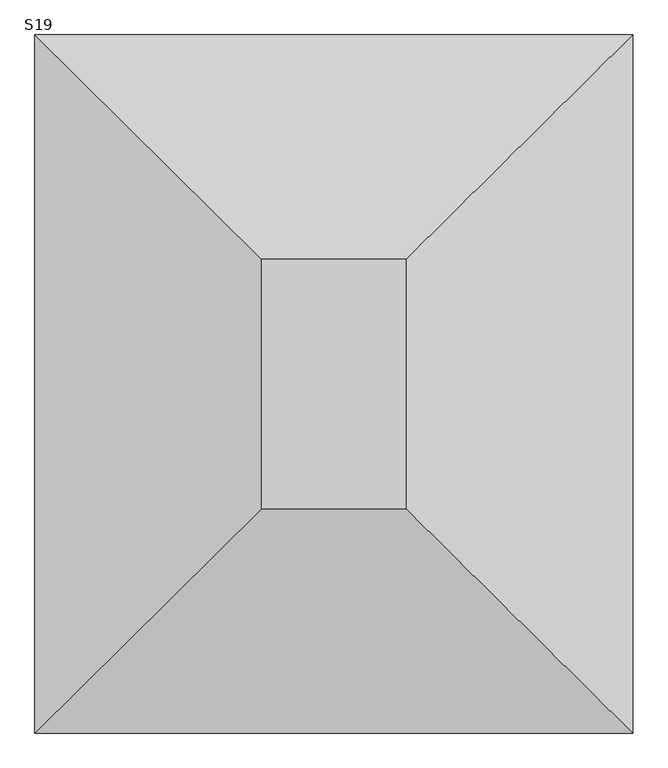
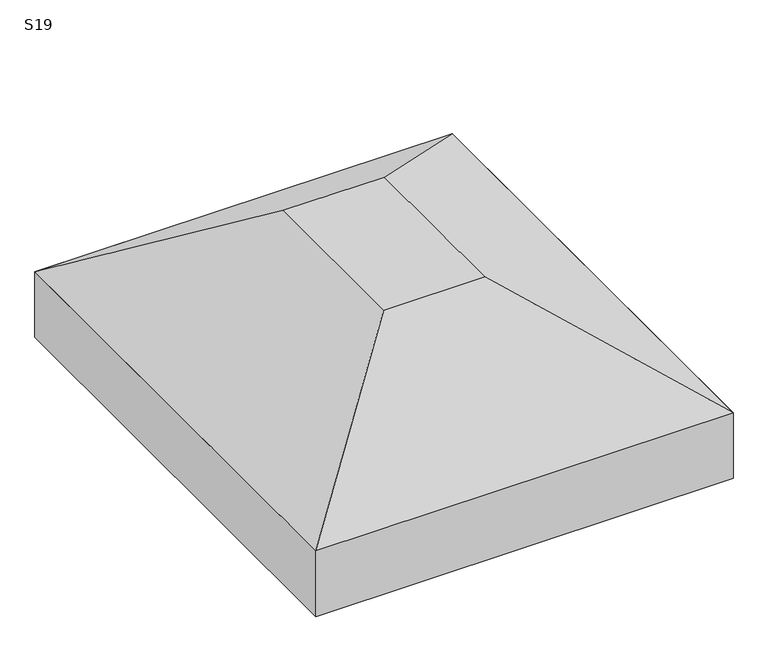
"""IFC4 building model written with IfcOpenShell, lengths in millimetres: fastener geometry, TQS - Sapata : S19."""

from ifc_helpers import new_model, si_unit, frame, origin, place, context, project, spatial, polyline, outline, extrude, faceted_brep, source, transform, mapped, element, save


def s19_c62a4a8b(model_context):
    return source(origin(), model_context, "Body", "SolidModel", [
        faceted_brep([(-55.0, 50.0, 0.0), (-345.0, 50.0, 0.0), (-345.0, -450.0, 0.0), (-55.0, -450.0, 0.0), (400.0, 500.0, -300.0), (400.0, -900.0, -300.0), (-800.0, -900.0, -300.0), (-800.0, 500.0, -300.0)], [[[0, 1, 2, 3]], [[4, 5, 6, 7]], [[4, 7, 1, 0]], [[7, 6, 2, 1]], [[6, 5, 3, 2]], [[5, 4, 0, 3]]]),
        extrude(outline(polyline([(400.0, 500.0), (400.0, -900.0), (-800.0, -900.0), (-800.0, 500.0), (400.0, 500.0)])), frame((0.0, 0.0, -500.0), z_axis=(0.0, 0.0, 1.0), x_axis=(1.0, 0.0, 0.0)), (0.0, 0.0, 1.0), 200.0),
    ])


if __name__ == "__main__":
    model = new_model("IFC4")
    model_context = context("Model", 3, world=origin())
    ifc_project = project(units=[si_unit("LENGTHUNIT", "METRE", prefix="MILLI")], contexts=[model_context])
    site = spatial("IfcSite", under=ifc_project)
    building = spatial("IfcBuilding", under=site)
    placement = place(None, origin())
    s19_shape = s19_c62a4a8b(model_context)
    element("IfcFastener", 1, ObjectType="TQS - Sapata : S19", at=placement, inside=building, context=model_context, shape_type="MappedRepresentation", body=[
        mapped(s19_shape, transform((0.0, 0.0, 0.0), x_axis=(1.0, 0.0, 0.0), y_axis=(0.0, 1.0, 0.0), z_axis=(0.0, 0.0, 1.0))),
    ])
    save(model, "model.ifc")

# Revit data of these elements
# Type "TQS - Sapata : S19"
#   TY = 0.50 m
#   TX = 0.29 m
#   HS = 0.50 m
#   H0 = 0.20 m
#   EXCYABS = 0.70 m
#   EXCY = 0.00 m
#   EXCXABS = 0.60 m
#   EXCX = 0.00 m
#   DIMY = 1.40 m
#   DIMX = 1.20 m
#   Material estrutural = Concreto - Concreto concretado no local
#   Width = 0
#   Length = 0
# Element 1 (IfcFastener, "TQS - Sapata : S19")
#   Materials on its faces: "Concreto - Concreto concretado no local"
# Materials
#   "Concreto - Concreto concretado no local": class "Concreto", colour RGB 192 192 192, transparency 0
